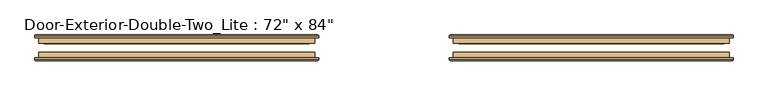
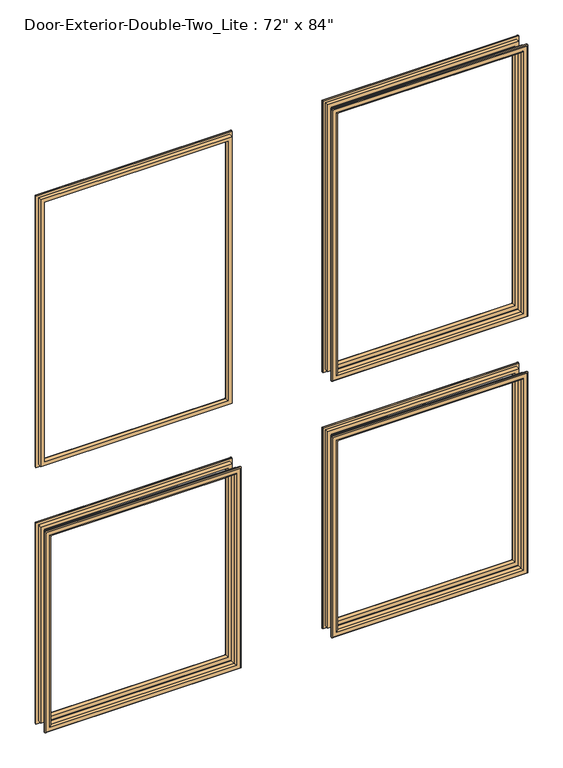
"""IFC4 building model written with IfcOpenShell, lengths in millimetres: door geometry."""

from ifc_helpers import new_model, si_unit, frame, origin, place, context, project, spatial, ellipse_curve, source, transform, mapped, element, save
from ifc_brep_helpers import plane_surface, cylinder_surface, advanced_brep


def door_a30fd648(model_context):
    return source(origin(), model_context, "Body", "AdvancedBrep", [
        advanced_brep(
        [(-762.0, 71.4375, 914.4), (-762.0, 84.1375, 914.4), (-762.0, 84.1375, 254.0), (-762.0, 71.4375, 254.0), (-750.0, 85.1375, 902.4), (-750.0, 71.4375, 902.4), (-750.0, 71.4375, 266.0), (-750.0, 85.1375, 266.0), (-755.0, 90.1375, 907.4), (-755.0, 90.1375, 261.0), (-770.0, 88.1375, 922.4), (-768.0, 90.1375, 920.4), (-768.0, 90.1375, 248.0), (-770.0, 88.1375, 246.0), (-770.0, 84.1375, 922.4), (-770.0, 84.1375, 246.0), (-152.4, 84.1375, 254.0), (-152.4, 71.4375, 254.0), (-164.4, 71.4375, 266.0), (-164.4, 85.1375, 266.0), (-159.4, 90.1375, 261.0), (-146.4, 90.1375, 248.0), (-144.4, 88.1375, 246.0), (-144.4, 84.1375, 246.0), (-152.4, 84.1375, 914.4), (-152.4, 71.4375, 914.4), (-164.4, 71.4375, 902.4), (-164.4, 85.1375, 902.4), (-159.4, 90.1375, 907.4), (-146.4, 90.1375, 920.4), (-144.4, 88.1375, 922.4), (-144.4, 84.1375, 922.4)],
        [
            (0, 1),
            (1, 2),
            (2, 3),
            (3, 0),
            (4, 5),
            (5, 6),
            (6, 7),
            (7, 4),
            (8, 4, ellipse_curve(frame((-755.0, 85.1375, 907.4), z_axis=(-0.7071067811865475, 0.0, -0.7071067811865475), x_axis=(-0.7071067811865474, 0.0, 0.7071067811865476)), 7.0710678, 5.0)),
            (7, 9, ellipse_curve(frame((-755.0, 85.1375, 261.0), z_axis=(-0.7071067811865475, 0.0, 0.7071067811865475), x_axis=(0.7071067811865474, 0.0, 0.7071067811865476)), 7.0710678, 5.0)),
            (9, 8),
            (10, 11, ellipse_curve(frame((-768.0, 88.1375, 920.4), z_axis=(-0.7071067811865475, 0.0, -0.7071067811865475), x_axis=(-0.7071067811865474, 0.0, 0.7071067811865476)), 2.8284271, 2.0)),
            (11, 12),
            (12, 13, ellipse_curve(frame((-768.0, 88.1375, 248.0), z_axis=(-0.7071067811865475, 0.0, 0.7071067811865475), x_axis=(0.7071067811865474, 0.0, 0.7071067811865476)), 2.8284271, 2.0)),
            (13, 10),
            (14, 10),
            (13, 15),
            (15, 14),
            (2, 16),
            (16, 17),
            (17, 3),
            (6, 18),
            (18, 19),
            (19, 7),
            (19, 20, ellipse_curve(frame((-159.4, 85.1375, 261.0), z_axis=(-0.7071067811865475, 0.0, -0.7071067811865475), x_axis=(-0.7071067811865476, 0.0, 0.7071067811865474)), 7.0710678, 5.0)),
            (20, 9),
            (12, 21),
            (21, 22, ellipse_curve(frame((-146.4, 88.1375, 248.0), z_axis=(-0.7071067811865475, 0.0, -0.7071067811865475), x_axis=(-0.7071067811865476, 0.0, 0.7071067811865474)), 2.8284271, 2.0)),
            (22, 13),
            (22, 23),
            (23, 15),
            (16, 24),
            (24, 25),
            (25, 17),
            (18, 26),
            (26, 27),
            (27, 19),
            (27, 28, ellipse_curve(frame((-159.4, 85.1375, 907.4), z_axis=(0.7071067811865475, 0.0, -0.7071067811865475), x_axis=(-0.7071067811865474, 0.0, -0.7071067811865476)), 7.0710678, 5.0)),
            (28, 20),
            (21, 29),
            (29, 30, ellipse_curve(frame((-146.4, 88.1375, 920.4), z_axis=(0.7071067811865475, 0.0, -0.7071067811865475), x_axis=(-0.7071067811865474, 0.0, -0.7071067811865476)), 2.8284271, 2.0)),
            (30, 22),
            (30, 31),
            (31, 23),
            (31, 14),
            (1, 24),
            (0, 25),
            (5, 26),
            (4, 27),
            (8, 28),
            (11, 29),
            (10, 30),
        ],
        [
            plane_surface(frame((-762.0, 84.1375, 914.4), z_axis=(-1.0, 0.0, 0.0), x_axis=(0.0, 0.0, -1.0))),
            plane_surface(frame((-750.0, 71.4375, 902.4), z_axis=(1.0, 0.0, 0.0), x_axis=(0.0, 0.0, -1.0))),
            cylinder_surface(frame((-755.0, 85.1375, 914.4), z_axis=(0.0, 0.0, 1.0), x_axis=(-1.0, 0.0, 0.0)), 5.0),
            cylinder_surface(frame((-768.0, 88.1375, 914.4), z_axis=(0.0, 0.0, 1.0), x_axis=(-1.0, 0.0, 0.0)), 2.0),
            plane_surface(frame((-770.0, 88.1375, 922.4), z_axis=(-1.0, 0.0, 0.0), x_axis=(0.0, 0.0, -1.0))),
            plane_surface(frame((-762.0, 84.1375, 254.0), z_axis=(0.0, 0.0, -1.0), x_axis=(1.0, 0.0, 0.0))),
            plane_surface(frame((-750.0, 71.4375, 266.0), z_axis=(0.0, 0.0, 1.0), x_axis=(1.0, 0.0, 0.0))),
            cylinder_surface(frame((-762.0, 85.1375, 261.0), z_axis=(-1.0, 0.0, 0.0), x_axis=(0.0, 0.0, -1.0)), 5.0),
            cylinder_surface(frame((-762.0, 88.1375, 248.0), z_axis=(-1.0, 0.0, 0.0), x_axis=(0.0, 0.0, -1.0)), 2.0),
            plane_surface(frame((-770.0, 88.1375, 246.0), z_axis=(0.0, 0.0, -1.0), x_axis=(1.0, 0.0, 0.0))),
            plane_surface(frame((-152.4, 84.1375, 254.0), z_axis=(1.0, 0.0, 0.0), x_axis=(0.0, 0.0, 1.0))),
            plane_surface(frame((-164.4, 71.4375, 266.0), z_axis=(-1.0, 0.0, 0.0), x_axis=(0.0, 0.0, 1.0))),
            cylinder_surface(frame((-159.4, 85.1375, 254.0), z_axis=(0.0, 0.0, -1.0), x_axis=(1.0, 0.0, 0.0)), 5.0),
            cylinder_surface(frame((-146.4, 88.1375, 254.0), z_axis=(0.0, 0.0, -1.0), x_axis=(1.0, 0.0, 0.0)), 2.0),
            plane_surface(frame((-144.4, 88.1375, 246.0), z_axis=(1.0, 0.0, 0.0), x_axis=(0.0, 0.0, 1.0))),
            plane_surface(frame((-144.4, 84.1375, 922.4), z_axis=(0.0, -1.0, 0.0), x_axis=(-1.0, 0.0, 0.0))),
            plane_surface(frame((-152.4, 84.1375, 914.4), z_axis=(0.0, 0.0, 1.0), x_axis=(-1.0, 0.0, 0.0))),
            plane_surface(frame((-152.4, 71.4375, 914.4), z_axis=(0.0, -1.0, 0.0), x_axis=(-1.0, 0.0, 0.0))),
            plane_surface(frame((-164.4, 71.4375, 902.4), z_axis=(0.0, 0.0, -1.0), x_axis=(-1.0, 0.0, 0.0))),
            cylinder_surface(frame((-152.4, 85.1375, 907.4), z_axis=(1.0, 0.0, 0.0), x_axis=(0.0, 0.0, 1.0)), 5.0),
            plane_surface(frame((-159.4, 90.1375, 907.4), z_axis=(0.0, 1.0, 0.0), x_axis=(-1.0, 0.0, 0.0))),
            cylinder_surface(frame((-152.4, 88.1375, 920.4), z_axis=(1.0, 0.0, 0.0), x_axis=(0.0, 0.0, 1.0)), 2.0),
            plane_surface(frame((-144.4, 88.1375, 922.4), z_axis=(0.0, 0.0, 1.0), x_axis=(-1.0, 0.0, 0.0))),
        ],
        [
            (0, [[1, 2, 3, 4]]),
            (1, [[5, 6, 7, 8]]),
            (2, [[9, -8, 10, 11]]),
            (3, [[12, 13, 14, 15]]),
            (4, [[16, -15, 17, 18]]),
            (5, [[-3, 19, 20, 21]]),
            (6, [[-7, 22, 23, 24]]),
            (7, [[-10, -24, 25, 26]]),
            (8, [[-14, 27, 28, 29]]),
            (9, [[-17, -29, 30, 31]]),
            (10, [[-20, 32, 33, 34]]),
            (11, [[-23, 35, 36, 37]]),
            (12, [[-25, -37, 38, 39]]),
            (13, [[-28, 40, 41, 42]]),
            (14, [[-30, -42, 43, 44]]),
            (15, [[-31, -44, 45, -18], [46, -32, -19, -2]]),
            (16, [[-33, -46, -1, 47]]),
            (17, [[-21, -34, -47, -4], [48, -35, -22, -6]]),
            (18, [[-36, -48, -5, 49]]),
            (19, [[-38, -49, -9, 50]]),
            (20, [[51, -40, -27, -13], [-26, -39, -50, -11]]),
            (21, [[-41, -51, -12, 52]]),
            (22, [[-43, -52, -16, -45]]),
        ],
    ),
        advanced_brep(
        [(152.4, 71.4375, 914.4), (152.4, 84.1375, 914.4), (152.4, 84.1375, 254.0), (152.4, 71.4375, 254.0), (164.4, 85.1375, 902.4), (164.4, 71.4375, 902.4), (164.4, 71.4375, 266.0), (164.4, 85.1375, 266.0), (159.4, 90.1375, 907.4), (159.4, 90.1375, 261.0), (144.4, 88.1375, 922.4), (146.4, 90.1375, 920.4), (146.4, 90.1375, 248.0), (144.4, 88.1375, 246.0), (144.4, 84.1375, 922.4), (144.4, 84.1375, 246.0), (762.0, 84.1375, 254.0), (762.0, 71.4375, 254.0), (750.0, 71.4375, 266.0), (750.0, 85.1375, 266.0), (755.0, 90.1375, 261.0), (768.0, 90.1375, 248.0), (770.0, 88.1375, 246.0), (770.0, 84.1375, 246.0), (762.0, 84.1375, 914.4), (762.0, 71.4375, 914.4), (750.0, 71.4375, 902.4), (750.0, 85.1375, 902.4), (755.0, 90.1375, 907.4), (768.0, 90.1375, 920.4), (770.0, 88.1375, 922.4), (770.0, 84.1375, 922.4)],
        [
            (0, 1),
            (1, 2),
            (2, 3),
            (3, 0),
            (4, 5),
            (5, 6),
            (6, 7),
            (7, 4),
            (8, 4, ellipse_curve(frame((159.4, 85.1375, 907.4), z_axis=(-0.7071067811865475, 0.0, -0.7071067811865475), x_axis=(-0.7071067811865474, 0.0, 0.7071067811865476)), 7.0710678, 5.0)),
            (7, 9, ellipse_curve(frame((159.4, 85.1375, 261.0), z_axis=(-0.7071067811865475, 0.0, 0.7071067811865475), x_axis=(0.7071067811865474, 0.0, 0.7071067811865476)), 7.0710678, 5.0)),
            (9, 8),
            (10, 11, ellipse_curve(frame((146.4, 88.1375, 920.4), z_axis=(-0.7071067811865475, 0.0, -0.7071067811865475), x_axis=(-0.7071067811865474, 0.0, 0.7071067811865476)), 2.8284271, 2.0)),
            (11, 12),
            (12, 13, ellipse_curve(frame((146.4, 88.1375, 248.0), z_axis=(-0.7071067811865475, 0.0, 0.7071067811865475), x_axis=(0.7071067811865474, 0.0, 0.7071067811865476)), 2.8284271, 2.0)),
            (13, 10),
            (14, 10),
            (13, 15),
            (15, 14),
            (2, 16),
            (16, 17),
            (17, 3),
            (6, 18),
            (18, 19),
            (19, 7),
            (19, 20, ellipse_curve(frame((755.0, 85.1375, 261.0), z_axis=(-0.7071067811865475, 0.0, -0.7071067811865475), x_axis=(-0.7071067811865476, 0.0, 0.7071067811865474)), 7.0710678, 5.0)),
            (20, 9),
            (12, 21),
            (21, 22, ellipse_curve(frame((768.0, 88.1375, 248.0), z_axis=(-0.7071067811865475, 0.0, -0.7071067811865475), x_axis=(-0.7071067811865476, 0.0, 0.7071067811865474)), 2.8284271, 2.0)),
            (22, 13),
            (22, 23),
            (23, 15),
            (16, 24),
            (24, 25),
            (25, 17),
            (18, 26),
            (26, 27),
            (27, 19),
            (27, 28, ellipse_curve(frame((755.0, 85.1375, 907.4), z_axis=(0.7071067811865475, 0.0, -0.7071067811865475), x_axis=(-0.7071067811865474, 0.0, -0.7071067811865476)), 7.0710678, 5.0)),
            (28, 20),
            (21, 29),
            (29, 30, ellipse_curve(frame((768.0, 88.1375, 920.4), z_axis=(0.7071067811865475, 0.0, -0.7071067811865475), x_axis=(-0.7071067811865474, 0.0, -0.7071067811865476)), 2.8284271, 2.0)),
            (30, 22),
            (30, 31),
            (31, 23),
            (31, 14),
            (1, 24),
            (0, 25),
            (5, 26),
            (4, 27),
            (8, 28),
            (11, 29),
            (10, 30),
        ],
        [
            plane_surface(frame((152.4, 84.1375, 914.4), z_axis=(-1.0, 0.0, 0.0), x_axis=(0.0, 0.0, -1.0))),
            plane_surface(frame((164.4, 71.4375, 902.4), z_axis=(1.0, 0.0, 0.0), x_axis=(0.0, 0.0, -1.0))),
            cylinder_surface(frame((159.4, 85.1375, 914.4), z_axis=(0.0, 0.0, 1.0), x_axis=(-1.0, 0.0, 0.0)), 5.0),
            cylinder_surface(frame((146.4, 88.1375, 914.4), z_axis=(0.0, 0.0, 1.0), x_axis=(-1.0, 0.0, 0.0)), 2.0),
            plane_surface(frame((144.4, 88.1375, 922.4), z_axis=(-1.0, 0.0, 0.0), x_axis=(0.0, 0.0, -1.0))),
            plane_surface(frame((152.4, 84.1375, 254.0), z_axis=(0.0, 0.0, -1.0), x_axis=(1.0, 0.0, 0.0))),
            plane_surface(frame((164.4, 71.4375, 266.0), z_axis=(0.0, 0.0, 1.0), x_axis=(1.0, 0.0, 0.0))),
            cylinder_surface(frame((152.4, 85.1375, 261.0), z_axis=(-1.0, 0.0, 0.0), x_axis=(0.0, 0.0, -1.0)), 5.0),
            cylinder_surface(frame((152.4, 88.1375, 248.0), z_axis=(-1.0, 0.0, 0.0), x_axis=(0.0, 0.0, -1.0)), 2.0),
            plane_surface(frame((144.4, 88.1375, 246.0), z_axis=(0.0, 0.0, -1.0), x_axis=(1.0, 0.0, 0.0))),
            plane_surface(frame((762.0, 84.1375, 254.0), z_axis=(1.0, 0.0, 0.0), x_axis=(0.0, 0.0, 1.0))),
            plane_surface(frame((750.0, 71.4375, 266.0), z_axis=(-1.0, 0.0, 0.0), x_axis=(0.0, 0.0, 1.0))),
            cylinder_surface(frame((755.0, 85.1375, 254.0), z_axis=(0.0, 0.0, -1.0), x_axis=(1.0, 0.0, 0.0)), 5.0),
            cylinder_surface(frame((768.0, 88.1375, 254.0), z_axis=(0.0, 0.0, -1.0), x_axis=(1.0, 0.0, 0.0)), 2.0),
            plane_surface(frame((770.0, 88.1375, 246.0), z_axis=(1.0, 0.0, 0.0), x_axis=(0.0, 0.0, 1.0))),
            plane_surface(frame((770.0, 84.1375, 922.4), z_axis=(0.0, -1.0, 0.0), x_axis=(-1.0, 0.0, 0.0))),
            plane_surface(frame((762.0, 84.1375, 914.4), z_axis=(0.0, 0.0, 1.0), x_axis=(-1.0, 0.0, 0.0))),
            plane_surface(frame((762.0, 71.4375, 914.4), z_axis=(0.0, -1.0, 0.0), x_axis=(-1.0, 0.0, 0.0))),
            plane_surface(frame((750.0, 71.4375, 902.4), z_axis=(0.0, 0.0, -1.0), x_axis=(-1.0, 0.0, 0.0))),
            cylinder_surface(frame((762.0, 85.1375, 907.4), z_axis=(1.0, 0.0, 0.0), x_axis=(0.0, 0.0, 1.0)), 5.0),
            plane_surface(frame((755.0, 90.1375, 907.4), z_axis=(0.0, 1.0, 0.0), x_axis=(-1.0, 0.0, 0.0))),
            cylinder_surface(frame((762.0, 88.1375, 920.4), z_axis=(1.0, 0.0, 0.0), x_axis=(0.0, 0.0, 1.0)), 2.0),
            plane_surface(frame((770.0, 88.1375, 922.4), z_axis=(0.0, 0.0, 1.0), x_axis=(-1.0, 0.0, 0.0))),
        ],
        [
            (0, [[1, 2, 3, 4]]),
            (1, [[5, 6, 7, 8]]),
            (2, [[9, -8, 10, 11]]),
            (3, [[12, 13, 14, 15]]),
            (4, [[16, -15, 17, 18]]),
            (5, [[-3, 19, 20, 21]]),
            (6, [[-7, 22, 23, 24]]),
            (7, [[-10, -24, 25, 26]]),
            (8, [[-14, 27, 28, 29]]),
            (9, [[-17, -29, 30, 31]]),
            (10, [[-20, 32, 33, 34]]),
            (11, [[-23, 35, 36, 37]]),
            (12, [[-25, -37, 38, 39]]),
            (13, [[-28, 40, 41, 42]]),
            (14, [[-30, -42, 43, 44]]),
            (15, [[-31, -44, 45, -18], [46, -32, -19, -2]]),
            (16, [[-33, -46, -1, 47]]),
            (17, [[-21, -34, -47, -4], [48, -35, -22, -6]]),
            (18, [[-36, -48, -5, 49]]),
            (19, [[-38, -49, -9, 50]]),
            (20, [[51, -40, -27, -13], [-26, -39, -50, -11]]),
            (21, [[-41, -51, -12, 52]]),
            (22, [[-43, -52, -16, -45]]),
        ],
    ),
        advanced_brep(
        [(152.4, 71.4375, 2016.125), (152.4, 84.1375, 2016.125), (152.4, 84.1375, 1117.6), (152.4, 71.4375, 1117.6), (164.4, 85.1375, 2004.125), (164.4, 71.4375, 2004.125), (164.4, 71.4375, 1129.6), (164.4, 85.1375, 1129.6), (159.4, 90.1375, 2009.125), (159.4, 90.1375, 1124.6), (144.4, 88.1375, 2024.125), (146.4, 90.1375, 2022.125), (146.4, 90.1375, 1111.6), (144.4, 88.1375, 1109.6), (144.4, 84.1375, 2024.125), (144.4, 84.1375, 1109.6), (762.0, 84.1375, 1117.6), (762.0, 71.4375, 1117.6), (750.0, 71.4375, 1129.6), (750.0, 85.1375, 1129.6), (755.0, 90.1375, 1124.6), (768.0, 90.1375, 1111.6), (770.0, 88.1375, 1109.6), (770.0, 84.1375, 1109.6), (762.0, 84.1375, 2016.125), (762.0, 71.4375, 2016.125), (750.0, 71.4375, 2004.125), (750.0, 85.1375, 2004.125), (755.0, 90.1375, 2009.125), (768.0, 90.1375, 2022.125), (770.0, 88.1375, 2024.125), (770.0, 84.1375, 2024.125)],
        [
            (0, 1),
            (1, 2),
            (2, 3),
            (3, 0),
            (4, 5),
            (5, 6),
            (6, 7),
            (7, 4),
            (8, 4, ellipse_curve(frame((159.4, 85.1375, 2009.125), z_axis=(-0.7071067811865475, 0.0, -0.7071067811865475), x_axis=(-0.7071067811865474, 0.0, 0.7071067811865476)), 7.0710678, 5.0)),
            (7, 9, ellipse_curve(frame((159.4, 85.1375, 1124.6), z_axis=(-0.7071067811865475, 0.0, 0.7071067811865475), x_axis=(0.7071067811865474, 0.0, 0.7071067811865476)), 7.0710678, 5.0)),
            (9, 8),
            (10, 11, ellipse_curve(frame((146.4, 88.1375, 2022.125), z_axis=(-0.7071067811865475, 0.0, -0.7071067811865475), x_axis=(-0.7071067811865474, 0.0, 0.7071067811865476)), 2.8284271, 2.0)),
            (11, 12),
            (12, 13, ellipse_curve(frame((146.4, 88.1375, 1111.6), z_axis=(-0.7071067811865475, 0.0, 0.7071067811865475), x_axis=(0.7071067811865474, 0.0, 0.7071067811865476)), 2.8284271, 2.0)),
            (13, 10),
            (14, 10),
            (13, 15),
            (15, 14),
            (2, 16),
            (16, 17),
            (17, 3),
            (6, 18),
            (18, 19),
            (19, 7),
            (19, 20, ellipse_curve(frame((755.0, 85.1375, 1124.6), z_axis=(-0.7071067811865475, 0.0, -0.7071067811865475), x_axis=(-0.7071067811865476, 0.0, 0.7071067811865474)), 7.0710678, 5.0)),
            (20, 9),
            (12, 21),
            (21, 22, ellipse_curve(frame((768.0, 88.1375, 1111.6), z_axis=(-0.7071067811865475, 0.0, -0.7071067811865475), x_axis=(-0.7071067811865476, 0.0, 0.7071067811865474)), 2.8284271, 2.0)),
            (22, 13),
            (22, 23),
            (23, 15),
            (16, 24),
            (24, 25),
            (25, 17),
            (18, 26),
            (26, 27),
            (27, 19),
            (27, 28, ellipse_curve(frame((755.0, 85.1375, 2009.125), z_axis=(0.7071067811865475, 0.0, -0.7071067811865475), x_axis=(-0.7071067811865474, 0.0, -0.7071067811865476)), 7.0710678, 5.0)),
            (28, 20),
            (21, 29),
            (29, 30, ellipse_curve(frame((768.0, 88.1375, 2022.125), z_axis=(0.7071067811865475, 0.0, -0.7071067811865475), x_axis=(-0.7071067811865474, 0.0, -0.7071067811865476)), 2.8284271, 2.0)),
            (30, 22),
            (30, 31),
            (31, 23),
            (31, 14),
            (1, 24),
            (0, 25),
            (5, 26),
            (4, 27),
            (8, 28),
            (11, 29),
            (10, 30),
        ],
        [
            plane_surface(frame((152.4, 84.1375, 2016.125), z_axis=(-1.0, 0.0, 0.0), x_axis=(0.0, 0.0, -1.0))),
            plane_surface(frame((164.4, 71.4375, 2004.125), z_axis=(1.0, 0.0, 0.0), x_axis=(0.0, 0.0, -1.0))),
            cylinder_surface(frame((159.4, 85.1375, 2016.125), z_axis=(0.0, 0.0, 1.0), x_axis=(-1.0, 0.0, 0.0)), 5.0),
            cylinder_surface(frame((146.4, 88.1375, 2016.125), z_axis=(0.0, 0.0, 1.0), x_axis=(-1.0, 0.0, 0.0)), 2.0),
            plane_surface(frame((144.4, 88.1375, 2024.125), z_axis=(-1.0, 0.0, 0.0), x_axis=(0.0, 0.0, -1.0))),
            plane_surface(frame((152.4, 84.1375, 1117.6), z_axis=(0.0, 0.0, -1.0), x_axis=(1.0, 0.0, 0.0))),
            plane_surface(frame((164.4, 71.4375, 1129.6), z_axis=(0.0, 0.0, 1.0), x_axis=(1.0, 0.0, 0.0))),
            cylinder_surface(frame((152.4, 85.1375, 1124.6), z_axis=(-1.0, 0.0, 0.0), x_axis=(0.0, 0.0, -1.0)), 5.0),
            cylinder_surface(frame((152.4, 88.1375, 1111.6), z_axis=(-1.0, 0.0, 0.0), x_axis=(0.0, 0.0, -1.0)), 2.0),
            plane_surface(frame((144.4, 88.1375, 1109.6), z_axis=(0.0, 0.0, -1.0), x_axis=(1.0, 0.0, 0.0))),
            plane_surface(frame((762.0, 84.1375, 1117.6), z_axis=(1.0, 0.0, 0.0), x_axis=(0.0, 0.0, 1.0))),
            plane_surface(frame((750.0, 71.4375, 1129.6), z_axis=(-1.0, 0.0, 0.0), x_axis=(0.0, 0.0, 1.0))),
            cylinder_surface(frame((755.0, 85.1375, 1117.6), z_axis=(0.0, 0.0, -1.0), x_axis=(1.0, 0.0, 0.0)), 5.0),
            cylinder_surface(frame((768.0, 88.1375, 1117.6), z_axis=(0.0, 0.0, -1.0), x_axis=(1.0, 0.0, 0.0)), 2.0),
            plane_surface(frame((770.0, 88.1375, 1109.6), z_axis=(1.0, 0.0, 0.0), x_axis=(0.0, 0.0, 1.0))),
            plane_surface(frame((770.0, 84.1375, 2024.125), z_axis=(0.0, -1.0, 0.0), x_axis=(-1.0, 0.0, 0.0))),
            plane_surface(frame((762.0, 84.1375, 2016.125), z_axis=(0.0, 0.0, 1.0), x_axis=(-1.0, 0.0, 0.0))),
            plane_surface(frame((762.0, 71.4375, 2016.125), z_axis=(0.0, -1.0, 0.0), x_axis=(-1.0, 0.0, 0.0))),
            plane_surface(frame((750.0, 71.4375, 2004.125), z_axis=(0.0, 0.0, -1.0), x_axis=(-1.0, 0.0, 0.0))),
            cylinder_surface(frame((762.0, 85.1375, 2009.125), z_axis=(1.0, 0.0, 0.0), x_axis=(0.0, 0.0, 1.0)), 5.0),
            plane_surface(frame((755.0, 90.1375, 2009.125), z_axis=(0.0, 1.0, 0.0), x_axis=(-1.0, 0.0, 0.0))),
            cylinder_surface(frame((762.0, 88.1375, 2022.125), z_axis=(1.0, 0.0, 0.0), x_axis=(0.0, 0.0, 1.0)), 2.0),
            plane_surface(frame((770.0, 88.1375, 2024.125), z_axis=(0.0, 0.0, 1.0), x_axis=(-1.0, 0.0, 0.0))),
        ],
        [
            (0, [[1, 2, 3, 4]]),
            (1, [[5, 6, 7, 8]]),
            (2, [[9, -8, 10, 11]]),
            (3, [[12, 13, 14, 15]]),
            (4, [[16, -15, 17, 18]]),
            (5, [[-3, 19, 20, 21]]),
            (6, [[-7, 22, 23, 24]]),
            (7, [[-10, -24, 25, 26]]),
            (8, [[-14, 27, 28, 29]]),
            (9, [[-17, -29, 30, 31]]),
            (10, [[-20, 32, 33, 34]]),
            (11, [[-23, 35, 36, 37]]),
            (12, [[-25, -37, 38, 39]]),
            (13, [[-28, 40, 41, 42]]),
            (14, [[-30, -42, 43, 44]]),
            (15, [[-31, -44, 45, -18], [46, -32, -19, -2]]),
            (16, [[-33, -46, -1, 47]]),
            (17, [[-21, -34, -47, -4], [48, -35, -22, -6]]),
            (18, [[-36, -48, -5, 49]]),
            (19, [[-38, -49, -9, 50]]),
            (20, [[51, -40, -27, -13], [-26, -39, -50, -11]]),
            (21, [[-41, -51, -12, 52]]),
            (22, [[-43, -52, -16, -45]]),
        ],
    ),
        advanced_brep(
        [(-762.0, 71.4375, 2016.125), (-762.0, 84.1375, 2016.125), (-762.0, 84.1375, 1117.6), (-762.0, 71.4375, 1117.6), (-750.0, 85.1375, 2004.125), (-750.0, 71.4375, 2004.125), (-750.0, 71.4375, 1129.6), (-750.0, 85.1375, 1129.6), (-755.0, 90.1375, 2009.125), (-755.0, 90.1375, 1124.6), (-770.0, 88.1375, 2024.125), (-768.0, 90.1375, 2022.125), (-768.0, 90.1375, 1111.6), (-770.0, 88.1375, 1109.6), (-770.0, 84.1375, 2024.125), (-770.0, 84.1375, 1109.6), (-152.4, 84.1375, 1117.6), (-152.4, 71.4375, 1117.6), (-164.4, 71.4375, 1129.6), (-164.4, 85.1375, 1129.6), (-159.4, 90.1375, 1124.6), (-146.4, 90.1375, 1111.6), (-144.4, 88.1375, 1109.6), (-144.4, 84.1375, 1109.6), (-152.4, 84.1375, 2016.125), (-152.4, 71.4375, 2016.125), (-164.4, 71.4375, 2004.125), (-164.4, 85.1375, 2004.125), (-159.4, 90.1375, 2009.125), (-146.4, 90.1375, 2022.125), (-144.4, 88.1375, 2024.125), (-144.4, 84.1375, 2024.125)],
        [
            (0, 1),
            (1, 2),
            (2, 3),
            (3, 0),
            (4, 5),
            (5, 6),
            (6, 7),
            (7, 4),
            (8, 4, ellipse_curve(frame((-755.0, 85.1375, 2009.125), z_axis=(-0.7071067811865475, 0.0, -0.7071067811865475), x_axis=(-0.7071067811865474, 0.0, 0.7071067811865476)), 7.0710678, 5.0)),
            (7, 9, ellipse_curve(frame((-755.0, 85.1375, 1124.6), z_axis=(-0.7071067811865475, 0.0, 0.7071067811865475), x_axis=(0.7071067811865474, 0.0, 0.7071067811865476)), 7.0710678, 5.0)),
            (9, 8),
            (10, 11, ellipse_curve(frame((-768.0, 88.1375, 2022.125), z_axis=(-0.7071067811865475, 0.0, -0.7071067811865475), x_axis=(-0.7071067811865474, 0.0, 0.7071067811865476)), 2.8284271, 2.0)),
            (11, 12),
            (12, 13, ellipse_curve(frame((-768.0, 88.1375, 1111.6), z_axis=(-0.7071067811865475, 0.0, 0.7071067811865475), x_axis=(0.7071067811865474, 0.0, 0.7071067811865476)), 2.8284271, 2.0)),
            (13, 10),
            (14, 10),
            (13, 15),
            (15, 14),
            (2, 16),
            (16, 17),
            (17, 3),
            (6, 18),
            (18, 19),
            (19, 7),
            (19, 20, ellipse_curve(frame((-159.4, 85.1375, 1124.6), z_axis=(-0.7071067811865475, 0.0, -0.7071067811865475), x_axis=(-0.7071067811865476, 0.0, 0.7071067811865474)), 7.0710678, 5.0)),
            (20, 9),
            (12, 21),
            (21, 22, ellipse_curve(frame((-146.4, 88.1375, 1111.6), z_axis=(-0.7071067811865475, 0.0, -0.7071067811865475), x_axis=(-0.7071067811865476, 0.0, 0.7071067811865474)), 2.8284271, 2.0)),
            (22, 13),
            (22, 23),
            (23, 15),
            (16, 24),
            (24, 25),
            (25, 17),
            (18, 26),
            (26, 27),
            (27, 19),
            (27, 28, ellipse_curve(frame((-159.4, 85.1375, 2009.125), z_axis=(0.7071067811865475, 0.0, -0.7071067811865475), x_axis=(-0.7071067811865474, 0.0, -0.7071067811865476)), 7.0710678, 5.0)),
            (28, 20),
            (21, 29),
            (29, 30, ellipse_curve(frame((-146.4, 88.1375, 2022.125), z_axis=(0.7071067811865475, 0.0, -0.7071067811865475), x_axis=(-0.7071067811865474, 0.0, -0.7071067811865476)), 2.8284271, 2.0)),
            (30, 22),
            (30, 31),
            (31, 23),
            (31, 14),
            (1, 24),
            (0, 25),
            (5, 26),
            (4, 27),
            (8, 28),
            (11, 29),
            (10, 30),
        ],
        [
            plane_surface(frame((-762.0, 84.1375, 2016.125), z_axis=(-1.0, 0.0, 0.0), x_axis=(0.0, 0.0, -1.0))),
            plane_surface(frame((-750.0, 71.4375, 2004.125), z_axis=(1.0, 0.0, 0.0), x_axis=(0.0, 0.0, -1.0))),
            cylinder_surface(frame((-755.0, 85.1375, 2016.125), z_axis=(0.0, 0.0, 1.0), x_axis=(-1.0, 0.0, 0.0)), 5.0),
            cylinder_surface(frame((-768.0, 88.1375, 2016.125), z_axis=(0.0, 0.0, 1.0), x_axis=(-1.0, 0.0, 0.0)), 2.0),
            plane_surface(frame((-770.0, 88.1375, 2024.125), z_axis=(-1.0, 0.0, 0.0), x_axis=(0.0, 0.0, -1.0))),
            plane_surface(frame((-762.0, 84.1375, 1117.6), z_axis=(0.0, 0.0, -1.0), x_axis=(1.0, 0.0, 0.0))),
            plane_surface(frame((-750.0, 71.4375, 1129.6), z_axis=(0.0, 0.0, 1.0), x_axis=(1.0, 0.0, 0.0))),
            cylinder_surface(frame((-762.0, 85.1375, 1124.6), z_axis=(-1.0, 0.0, 0.0), x_axis=(0.0, 0.0, -1.0)), 5.0),
            cylinder_surface(frame((-762.0, 88.1375, 1111.6), z_axis=(-1.0, 0.0, 0.0), x_axis=(0.0, 0.0, -1.0)), 2.0),
            plane_surface(frame((-770.0, 88.1375, 1109.6), z_axis=(0.0, 0.0, -1.0), x_axis=(1.0, 0.0, 0.0))),
            plane_surface(frame((-152.4, 84.1375, 1117.6), z_axis=(1.0, 0.0, 0.0), x_axis=(0.0, 0.0, 1.0))),
            plane_surface(frame((-164.4, 71.4375, 1129.6), z_axis=(-1.0, 0.0, 0.0), x_axis=(0.0, 0.0, 1.0))),
            cylinder_surface(frame((-159.4, 85.1375, 1117.6), z_axis=(0.0, 0.0, -1.0), x_axis=(1.0, 0.0, 0.0)), 5.0),
            cylinder_surface(frame((-146.4, 88.1375, 1117.6), z_axis=(0.0, 0.0, -1.0), x_axis=(1.0, 0.0, 0.0)), 2.0),
            plane_surface(frame((-144.4, 88.1375, 1109.6), z_axis=(1.0, 0.0, 0.0), x_axis=(0.0, 0.0, 1.0))),
            plane_surface(frame((-144.4, 84.1375, 2024.125), z_axis=(0.0, -1.0, 0.0), x_axis=(-1.0, 0.0, 0.0))),
            plane_surface(frame((-152.4, 84.1375, 2016.125), z_axis=(0.0, 0.0, 1.0), x_axis=(-1.0, 0.0, 0.0))),
            plane_surface(frame((-152.4, 71.4375, 2016.125), z_axis=(0.0, -1.0, 0.0), x_axis=(-1.0, 0.0, 0.0))),
            plane_surface(frame((-164.4, 71.4375, 2004.125), z_axis=(0.0, 0.0, -1.0), x_axis=(-1.0, 0.0, 0.0))),
            cylinder_surface(frame((-152.4, 85.1375, 2009.125), z_axis=(1.0, 0.0, 0.0), x_axis=(0.0, 0.0, 1.0)), 5.0),
            plane_surface(frame((-159.4, 90.1375, 2009.125), z_axis=(0.0, 1.0, 0.0), x_axis=(-1.0, 0.0, 0.0))),
            cylinder_surface(frame((-152.4, 88.1375, 2022.125), z_axis=(1.0, 0.0, 0.0), x_axis=(0.0, 0.0, 1.0)), 2.0),
            plane_surface(frame((-144.4, 88.1375, 2024.125), z_axis=(0.0, 0.0, 1.0), x_axis=(-1.0, 0.0, 0.0))),
        ],
        [
            (0, [[1, 2, 3, 4]]),
            (1, [[5, 6, 7, 8]]),
            (2, [[9, -8, 10, 11]]),
            (3, [[12, 13, 14, 15]]),
            (4, [[16, -15, 17, 18]]),
            (5, [[-3, 19, 20, 21]]),
            (6, [[-7, 22, 23, 24]]),
            (7, [[-10, -24, 25, 26]]),
            (8, [[-14, 27, 28, 29]]),
            (9, [[-17, -29, 30, 31]]),
            (10, [[-20, 32, 33, 34]]),
            (11, [[-23, 35, 36, 37]]),
            (12, [[-25, -37, 38, 39]]),
            (13, [[-28, 40, 41, 42]]),
            (14, [[-30, -42, 43, 44]]),
            (15, [[-31, -44, 45, -18], [46, -32, -19, -2]]),
            (16, [[-33, -46, -1, 47]]),
            (17, [[-21, -34, -47, -4], [48, -35, -22, -6]]),
            (18, [[-36, -48, -5, 49]]),
            (19, [[-38, -49, -9, 50]]),
            (20, [[51, -40, -27, -13], [-26, -39, -50, -11]]),
            (21, [[-41, -51, -12, 52]]),
            (22, [[-43, -52, -16, -45]]),
        ],
    ),
        advanced_brep(
        [(-762.0, 52.3875, 254.0), (-762.0, 39.6875, 254.0), (-762.0, 39.6875, 914.4), (-762.0, 52.3875, 914.4), (-750.0, 38.6875, 266.0), (-750.0, 52.3875, 266.0), (-750.0, 52.3875, 902.4), (-750.0, 38.6875, 902.4), (-755.0, 33.6875, 261.0), (-755.0, 33.6875, 907.4), (-770.0, 35.6875, 246.0), (-768.0, 33.6875, 248.0), (-768.0, 33.6875, 920.4), (-770.0, 35.6875, 922.4), (-770.0, 39.6875, 246.0), (-770.0, 39.6875, 922.4), (-152.4, 39.6875, 914.4), (-152.4, 52.3875, 914.4), (-164.4, 52.3875, 902.4), (-164.4, 38.6875, 902.4), (-159.4, 33.6875, 907.4), (-146.4, 33.6875, 920.4), (-144.4, 35.6875, 922.4), (-144.4, 39.6875, 922.4), (-152.4, 39.6875, 254.0), (-152.4, 52.3875, 254.0), (-164.4, 52.3875, 266.0), (-164.4, 38.6875, 266.0), (-159.4, 33.6875, 261.0), (-146.4, 33.6875, 248.0), (-144.4, 35.6875, 246.0), (-144.4, 39.6875, 246.0)],
        [
            (0, 1),
            (1, 2),
            (2, 3),
            (3, 0),
            (4, 5),
            (5, 6),
            (6, 7),
            (7, 4),
            (8, 4, ellipse_curve(frame((-755.0, 38.6875, 261.0), z_axis=(-0.7071067811865475, 0.0, 0.7071067811865475), x_axis=(-0.7071067811865474, 0.0, -0.7071067811865476)), 7.0710678, 5.0)),
            (7, 9, ellipse_curve(frame((-755.0, 38.6875, 907.4), z_axis=(-0.7071067811865475, 0.0, -0.7071067811865475), x_axis=(0.7071067811865474, 0.0, -0.7071067811865476)), 7.0710678, 5.0)),
            (9, 8),
            (10, 11, ellipse_curve(frame((-768.0, 35.6875, 248.0), z_axis=(-0.7071067811865475, 0.0, 0.7071067811865475), x_axis=(-0.7071067811865474, 0.0, -0.7071067811865476)), 2.8284271, 2.0)),
            (11, 12),
            (12, 13, ellipse_curve(frame((-768.0, 35.6875, 920.4), z_axis=(-0.7071067811865475, 0.0, -0.7071067811865475), x_axis=(0.7071067811865474, 0.0, -0.7071067811865476)), 2.8284271, 2.0)),
            (13, 10),
            (14, 10),
            (13, 15),
            (15, 14),
            (2, 16),
            (16, 17),
            (17, 3),
            (6, 18),
            (18, 19),
            (19, 7),
            (19, 20, ellipse_curve(frame((-159.4, 38.6875, 907.4), z_axis=(-0.7071067811865475, 0.0, 0.7071067811865475), x_axis=(-0.7071067811865476, 0.0, -0.7071067811865474)), 7.0710678, 5.0)),
            (20, 9),
            (12, 21),
            (21, 22, ellipse_curve(frame((-146.4, 35.6875, 920.4), z_axis=(-0.7071067811865475, 0.0, 0.7071067811865475), x_axis=(-0.7071067811865476, 0.0, -0.7071067811865474)), 2.8284271, 2.0)),
            (22, 13),
            (22, 23),
            (23, 15),
            (16, 24),
            (24, 25),
            (25, 17),
            (18, 26),
            (26, 27),
            (27, 19),
            (27, 28, ellipse_curve(frame((-159.4, 38.6875, 261.0), z_axis=(0.7071067811865475, 0.0, 0.7071067811865475), x_axis=(-0.7071067811865474, 0.0, 0.7071067811865476)), 7.0710678, 5.0)),
            (28, 20),
            (21, 29),
            (29, 30, ellipse_curve(frame((-146.4, 35.6875, 248.0), z_axis=(0.7071067811865475, 0.0, 0.7071067811865475), x_axis=(-0.7071067811865474, 0.0, 0.7071067811865476)), 2.8284271, 2.0)),
            (30, 22),
            (30, 31),
            (31, 23),
            (31, 14),
            (1, 24),
            (0, 25),
            (5, 26),
            (4, 27),
            (8, 28),
            (11, 29),
            (10, 30),
        ],
        [
            plane_surface(frame((-762.0, 39.6875, 254.0), z_axis=(-1.0, 0.0, 0.0), x_axis=(0.0, 0.0, 1.0))),
            plane_surface(frame((-750.0, 52.3875, 266.0), z_axis=(1.0, 0.0, 0.0), x_axis=(0.0, 0.0, 1.0))),
            cylinder_surface(frame((-755.0, 38.6875, 254.0), z_axis=(0.0, 0.0, -1.0), x_axis=(-1.0, 0.0, 0.0)), 5.0),
            cylinder_surface(frame((-768.0, 35.6875, 254.0), z_axis=(0.0, 0.0, -1.0), x_axis=(-1.0, 0.0, 0.0)), 2.0),
            plane_surface(frame((-770.0, 35.6875, 246.0), z_axis=(-1.0, 0.0, 0.0), x_axis=(0.0, 0.0, 1.0))),
            plane_surface(frame((-762.0, 39.6875, 914.4), z_axis=(0.0, 0.0, 1.0), x_axis=(1.0, 0.0, 0.0))),
            plane_surface(frame((-750.0, 52.3875, 902.4), z_axis=(0.0, 0.0, -1.0), x_axis=(1.0, 0.0, 0.0))),
            cylinder_surface(frame((-762.0, 38.6875, 907.4), z_axis=(-1.0, 0.0, 0.0), x_axis=(0.0, 0.0, 1.0)), 5.0),
            cylinder_surface(frame((-762.0, 35.6875, 920.4), z_axis=(-1.0, 0.0, 0.0), x_axis=(0.0, 0.0, 1.0)), 2.0),
            plane_surface(frame((-770.0, 35.6875, 922.4), z_axis=(0.0, 0.0, 1.0), x_axis=(1.0, 0.0, 0.0))),
            plane_surface(frame((-152.4, 39.6875, 914.4), z_axis=(1.0, 0.0, 0.0), x_axis=(0.0, 0.0, -1.0))),
            plane_surface(frame((-164.4, 52.3875, 902.4), z_axis=(-1.0, 0.0, 0.0), x_axis=(0.0, 0.0, -1.0))),
            cylinder_surface(frame((-159.4, 38.6875, 914.4), z_axis=(0.0, 0.0, 1.0), x_axis=(1.0, 0.0, 0.0)), 5.0),
            cylinder_surface(frame((-146.4, 35.6875, 914.4), z_axis=(0.0, 0.0, 1.0), x_axis=(1.0, 0.0, 0.0)), 2.0),
            plane_surface(frame((-144.4, 35.6875, 922.4), z_axis=(1.0, 0.0, 0.0), x_axis=(0.0, 0.0, -1.0))),
            plane_surface(frame((-144.4, 39.6875, 246.0), z_axis=(0.0, 1.0, 0.0), x_axis=(-1.0, 0.0, 0.0))),
            plane_surface(frame((-152.4, 39.6875, 254.0), z_axis=(0.0, 0.0, -1.0), x_axis=(-1.0, 0.0, 0.0))),
            plane_surface(frame((-152.4, 52.3875, 254.0), z_axis=(0.0, 1.0, 0.0), x_axis=(-1.0, 0.0, 0.0))),
            plane_surface(frame((-164.4, 52.3875, 266.0), z_axis=(0.0, 0.0, 1.0), x_axis=(-1.0, 0.0, 0.0))),
            cylinder_surface(frame((-152.4, 38.6875, 261.0), z_axis=(1.0, 0.0, 0.0), x_axis=(0.0, 0.0, -1.0)), 5.0),
            plane_surface(frame((-159.4, 33.6875, 261.0), z_axis=(0.0, -1.0, 0.0), x_axis=(-1.0, 0.0, 0.0))),
            cylinder_surface(frame((-152.4, 35.6875, 248.0), z_axis=(1.0, 0.0, 0.0), x_axis=(0.0, 0.0, -1.0)), 2.0),
            plane_surface(frame((-144.4, 35.6875, 246.0), z_axis=(0.0, 0.0, -1.0), x_axis=(-1.0, 0.0, 0.0))),
        ],
        [
            (0, [[1, 2, 3, 4]]),
            (1, [[5, 6, 7, 8]]),
            (2, [[9, -8, 10, 11]]),
            (3, [[12, 13, 14, 15]]),
            (4, [[16, -15, 17, 18]]),
            (5, [[-3, 19, 20, 21]]),
            (6, [[-7, 22, 23, 24]]),
            (7, [[-10, -24, 25, 26]]),
            (8, [[-14, 27, 28, 29]]),
            (9, [[-17, -29, 30, 31]]),
            (10, [[-20, 32, 33, 34]]),
            (11, [[-23, 35, 36, 37]]),
            (12, [[-25, -37, 38, 39]]),
            (13, [[-28, 40, 41, 42]]),
            (14, [[-30, -42, 43, 44]]),
            (15, [[-31, -44, 45, -18], [46, -32, -19, -2]]),
            (16, [[-33, -46, -1, 47]]),
            (17, [[-21, -34, -47, -4], [48, -35, -22, -6]]),
            (18, [[-36, -48, -5, 49]]),
            (19, [[-38, -49, -9, 50]]),
            (20, [[51, -40, -27, -13], [-26, -39, -50, -11]]),
            (21, [[-41, -51, -12, 52]]),
            (22, [[-43, -52, -16, -45]]),
        ],
    ),
        advanced_brep(
        [(152.4, 52.3875, 254.0), (152.4, 39.6875, 254.0), (152.4, 39.6875, 914.4), (152.4, 52.3875, 914.4), (164.4, 38.6875, 266.0), (164.4, 52.3875, 266.0), (164.4, 52.3875, 902.4), (164.4, 38.6875, 902.4), (159.4, 33.6875, 261.0), (159.4, 33.6875, 907.4), (144.4, 35.6875, 246.0), (146.4, 33.6875, 248.0), (146.4, 33.6875, 920.4), (144.4, 35.6875, 922.4), (144.4, 39.6875, 246.0), (144.4, 39.6875, 922.4), (762.0, 39.6875, 914.4), (762.0, 52.3875, 914.4), (750.0, 52.3875, 902.4), (750.0, 38.6875, 902.4), (755.0, 33.6875, 907.4), (768.0, 33.6875, 920.4), (770.0, 35.6875, 922.4), (770.0, 39.6875, 922.4), (762.0, 39.6875, 254.0), (762.0, 52.3875, 254.0), (750.0, 52.3875, 266.0), (750.0, 38.6875, 266.0), (755.0, 33.6875, 261.0), (768.0, 33.6875, 248.0), (770.0, 35.6875, 246.0), (770.0, 39.6875, 246.0)],
        [
            (0, 1),
            (1, 2),
            (2, 3),
            (3, 0),
            (4, 5),
            (5, 6),
            (6, 7),
            (7, 4),
            (8, 4, ellipse_curve(frame((159.4, 38.6875, 261.0), z_axis=(-0.7071067811865475, 0.0, 0.7071067811865475), x_axis=(-0.7071067811865474, 0.0, -0.7071067811865476)), 7.0710678, 5.0)),
            (7, 9, ellipse_curve(frame((159.4, 38.6875, 907.4), z_axis=(-0.7071067811865475, 0.0, -0.7071067811865475), x_axis=(0.7071067811865474, 0.0, -0.7071067811865476)), 7.0710678, 5.0)),
            (9, 8),
            (10, 11, ellipse_curve(frame((146.4, 35.6875, 248.0), z_axis=(-0.7071067811865475, 0.0, 0.7071067811865475), x_axis=(-0.7071067811865474, 0.0, -0.7071067811865476)), 2.8284271, 2.0)),
            (11, 12),
            (12, 13, ellipse_curve(frame((146.4, 35.6875, 920.4), z_axis=(-0.7071067811865475, 0.0, -0.7071067811865475), x_axis=(0.7071067811865474, 0.0, -0.7071067811865476)), 2.8284271, 2.0)),
            (13, 10),
            (14, 10),
            (13, 15),
            (15, 14),
            (2, 16),
            (16, 17),
            (17, 3),
            (6, 18),
            (18, 19),
            (19, 7),
            (19, 20, ellipse_curve(frame((755.0, 38.6875, 907.4), z_axis=(-0.7071067811865475, 0.0, 0.7071067811865475), x_axis=(-0.7071067811865476, 0.0, -0.7071067811865474)), 7.0710678, 5.0)),
            (20, 9),
            (12, 21),
            (21, 22, ellipse_curve(frame((768.0, 35.6875, 920.4), z_axis=(-0.7071067811865475, 0.0, 0.7071067811865475), x_axis=(-0.7071067811865476, 0.0, -0.7071067811865474)), 2.8284271, 2.0)),
            (22, 13),
            (22, 23),
            (23, 15),
            (16, 24),
            (24, 25),
            (25, 17),
            (18, 26),
            (26, 27),
            (27, 19),
            (27, 28, ellipse_curve(frame((755.0, 38.6875, 261.0), z_axis=(0.7071067811865475, 0.0, 0.7071067811865475), x_axis=(-0.7071067811865474, 0.0, 0.7071067811865476)), 7.0710678, 5.0)),
            (28, 20),
            (21, 29),
            (29, 30, ellipse_curve(frame((768.0, 35.6875, 248.0), z_axis=(0.7071067811865475, 0.0, 0.7071067811865475), x_axis=(-0.7071067811865474, 0.0, 0.7071067811865476)), 2.8284271, 2.0)),
            (30, 22),
            (30, 31),
            (31, 23),
            (31, 14),
            (1, 24),
            (0, 25),
            (5, 26),
            (4, 27),
            (8, 28),
            (11, 29),
            (10, 30),
        ],
        [
            plane_surface(frame((152.4, 39.6875, 254.0), z_axis=(-1.0, 0.0, 0.0), x_axis=(0.0, 0.0, 1.0))),
            plane_surface(frame((164.4, 52.3875, 266.0), z_axis=(1.0, 0.0, 0.0), x_axis=(0.0, 0.0, 1.0))),
            cylinder_surface(frame((159.4, 38.6875, 254.0), z_axis=(0.0, 0.0, -1.0), x_axis=(-1.0, 0.0, 0.0)), 5.0),
            cylinder_surface(frame((146.4, 35.6875, 254.0), z_axis=(0.0, 0.0, -1.0), x_axis=(-1.0, 0.0, 0.0)), 2.0),
            plane_surface(frame((144.4, 35.6875, 246.0), z_axis=(-1.0, 0.0, 0.0), x_axis=(0.0, 0.0, 1.0))),
            plane_surface(frame((152.4, 39.6875, 914.4), z_axis=(0.0, 0.0, 1.0), x_axis=(1.0, 0.0, 0.0))),
            plane_surface(frame((164.4, 52.3875, 902.4), z_axis=(0.0, 0.0, -1.0), x_axis=(1.0, 0.0, 0.0))),
            cylinder_surface(frame((152.4, 38.6875, 907.4), z_axis=(-1.0, 0.0, 0.0), x_axis=(0.0, 0.0, 1.0)), 5.0),
            cylinder_surface(frame((152.4, 35.6875, 920.4), z_axis=(-1.0, 0.0, 0.0), x_axis=(0.0, 0.0, 1.0)), 2.0),
            plane_surface(frame((144.4, 35.6875, 922.4), z_axis=(0.0, 0.0, 1.0), x_axis=(1.0, 0.0, 0.0))),
            plane_surface(frame((762.0, 39.6875, 914.4), z_axis=(1.0, 0.0, 0.0), x_axis=(0.0, 0.0, -1.0))),
            plane_surface(frame((750.0, 52.3875, 902.4), z_axis=(-1.0, 0.0, 0.0), x_axis=(0.0, 0.0, -1.0))),
            cylinder_surface(frame((755.0, 38.6875, 914.4), z_axis=(0.0, 0.0, 1.0), x_axis=(1.0, 0.0, 0.0)), 5.0),
            cylinder_surface(frame((768.0, 35.6875, 914.4), z_axis=(0.0, 0.0, 1.0), x_axis=(1.0, 0.0, 0.0)), 2.0),
            plane_surface(frame((770.0, 35.6875, 922.4), z_axis=(1.0, 0.0, 0.0), x_axis=(0.0, 0.0, -1.0))),
            plane_surface(frame((770.0, 39.6875, 246.0), z_axis=(0.0, 1.0, 0.0), x_axis=(-1.0, 0.0, 0.0))),
            plane_surface(frame((762.0, 39.6875, 254.0), z_axis=(0.0, 0.0, -1.0), x_axis=(-1.0, 0.0, 0.0))),
            plane_surface(frame((762.0, 52.3875, 254.0), z_axis=(0.0, 1.0, 0.0), x_axis=(-1.0, 0.0, 0.0))),
            plane_surface(frame((750.0, 52.3875, 266.0), z_axis=(0.0, 0.0, 1.0), x_axis=(-1.0, 0.0, 0.0))),
            cylinder_surface(frame((762.0, 38.6875, 261.0), z_axis=(1.0, 0.0, 0.0), x_axis=(0.0, 0.0, -1.0)), 5.0),
            plane_surface(frame((755.0, 33.6875, 261.0), z_axis=(0.0, -1.0, 0.0), x_axis=(-1.0, 0.0, 0.0))),
            cylinder_surface(frame((762.0, 35.6875, 248.0), z_axis=(1.0, 0.0, 0.0), x_axis=(0.0, 0.0, -1.0)), 2.0),
            plane_surface(frame((770.0, 35.6875, 246.0), z_axis=(0.0, 0.0, -1.0), x_axis=(-1.0, 0.0, 0.0))),
        ],
        [
            (0, [[1, 2, 3, 4]]),
            (1, [[5, 6, 7, 8]]),
            (2, [[9, -8, 10, 11]]),
            (3, [[12, 13, 14, 15]]),
            (4, [[16, -15, 17, 18]]),
            (5, [[-3, 19, 20, 21]]),
            (6, [[-7, 22, 23, 24]]),
            (7, [[-10, -24, 25, 26]]),
            (8, [[-14, 27, 28, 29]]),
            (9, [[-17, -29, 30, 31]]),
            (10, [[-20, 32, 33, 34]]),
            (11, [[-23, 35, 36, 37]]),
            (12, [[-25, -37, 38, 39]]),
            (13, [[-28, 40, 41, 42]]),
            (14, [[-30, -42, 43, 44]]),
            (15, [[-31, -44, 45, -18], [46, -32, -19, -2]]),
            (16, [[-33, -46, -1, 47]]),
            (17, [[-21, -34, -47, -4], [48, -35, -22, -6]]),
            (18, [[-36, -48, -5, 49]]),
            (19, [[-38, -49, -9, 50]]),
            (20, [[51, -40, -27, -13], [-26, -39, -50, -11]]),
            (21, [[-41, -51, -12, 52]]),
            (22, [[-43, -52, -16, -45]]),
        ],
    ),
        advanced_brep(
        [(152.4, 52.3875, 1117.6), (152.4, 39.6875, 1117.6), (152.4, 39.6875, 2016.125), (152.4, 52.3875, 2016.125), (164.4, 38.6875, 1129.6), (164.4, 52.3875, 1129.6), (164.4, 52.3875, 2004.125), (164.4, 38.6875, 2004.125), (159.4, 33.6875, 1124.6), (159.4, 33.6875, 2009.125), (144.4, 35.6875, 1109.6), (146.4, 33.6875, 1111.6), (146.4, 33.6875, 2022.125), (144.4, 35.6875, 2024.125), (144.4, 39.6875, 1109.6), (144.4, 39.6875, 2024.125), (762.0, 39.6875, 2016.125), (762.0, 52.3875, 2016.125), (750.0, 52.3875, 2004.125), (750.0, 38.6875, 2004.125), (755.0, 33.6875, 2009.125), (768.0, 33.6875, 2022.125), (770.0, 35.6875, 2024.125), (770.0, 39.6875, 2024.125), (762.0, 39.6875, 1117.6), (762.0, 52.3875, 1117.6), (750.0, 52.3875, 1129.6), (750.0, 38.6875, 1129.6), (755.0, 33.6875, 1124.6), (768.0, 33.6875, 1111.6), (770.0, 35.6875, 1109.6), (770.0, 39.6875, 1109.6)],
        [
            (0, 1),
            (1, 2),
            (2, 3),
            (3, 0),
            (4, 5),
            (5, 6),
            (6, 7),
            (7, 4),
            (8, 4, ellipse_curve(frame((159.4, 38.6875, 1124.6), z_axis=(-0.7071067811865475, 0.0, 0.7071067811865475), x_axis=(-0.7071067811865474, 0.0, -0.7071067811865476)), 7.0710678, 5.0)),
            (7, 9, ellipse_curve(frame((159.4, 38.6875, 2009.125), z_axis=(-0.7071067811865475, 0.0, -0.7071067811865475), x_axis=(0.7071067811865474, 0.0, -0.7071067811865476)), 7.0710678, 5.0)),
            (9, 8),
            (10, 11, ellipse_curve(frame((146.4, 35.6875, 1111.6), z_axis=(-0.7071067811865475, 0.0, 0.7071067811865475), x_axis=(-0.7071067811865474, 0.0, -0.7071067811865476)), 2.8284271, 2.0)),
            (11, 12),
            (12, 13, ellipse_curve(frame((146.4, 35.6875, 2022.125), z_axis=(-0.7071067811865475, 0.0, -0.7071067811865475), x_axis=(0.7071067811865474, 0.0, -0.7071067811865476)), 2.8284271, 2.0)),
            (13, 10),
            (14, 10),
            (13, 15),
            (15, 14),
            (2, 16),
            (16, 17),
            (17, 3),
            (6, 18),
            (18, 19),
            (19, 7),
            (19, 20, ellipse_curve(frame((755.0, 38.6875, 2009.125), z_axis=(-0.7071067811865475, 0.0, 0.7071067811865475), x_axis=(-0.7071067811865476, 0.0, -0.7071067811865474)), 7.0710678, 5.0)),
            (20, 9),
            (12, 21),
            (21, 22, ellipse_curve(frame((768.0, 35.6875, 2022.125), z_axis=(-0.7071067811865475, 0.0, 0.7071067811865475), x_axis=(-0.7071067811865476, 0.0, -0.7071067811865474)), 2.8284271, 2.0)),
            (22, 13),
            (22, 23),
            (23, 15),
            (16, 24),
            (24, 25),
            (25, 17),
            (18, 26),
            (26, 27),
            (27, 19),
            (27, 28, ellipse_curve(frame((755.0, 38.6875, 1124.6), z_axis=(0.7071067811865475, 0.0, 0.7071067811865475), x_axis=(-0.7071067811865474, 0.0, 0.7071067811865476)), 7.0710678, 5.0)),
            (28, 20),
            (21, 29),
            (29, 30, ellipse_curve(frame((768.0, 35.6875, 1111.6), z_axis=(0.7071067811865475, 0.0, 0.7071067811865475), x_axis=(-0.7071067811865474, 0.0, 0.7071067811865476)), 2.8284271, 2.0)),
            (30, 22),
            (30, 31),
            (31, 23),
            (31, 14),
            (1, 24),
            (0, 25),
            (5, 26),
            (4, 27),
            (8, 28),
            (11, 29),
            (10, 30),
        ],
        [
            plane_surface(frame((152.4, 39.6875, 1117.6), z_axis=(-1.0, 0.0, 0.0), x_axis=(0.0, 0.0, 1.0))),
            plane_surface(frame((164.4, 52.3875, 1129.6), z_axis=(1.0, 0.0, 0.0), x_axis=(0.0, 0.0, 1.0))),
            cylinder_surface(frame((159.4, 38.6875, 1117.6), z_axis=(0.0, 0.0, -1.0), x_axis=(-1.0, 0.0, 0.0)), 5.0),
            cylinder_surface(frame((146.4, 35.6875, 1117.6), z_axis=(0.0, 0.0, -1.0), x_axis=(-1.0, 0.0, 0.0)), 2.0),
            plane_surface(frame((144.4, 35.6875, 1109.6), z_axis=(-1.0, 0.0, 0.0), x_axis=(0.0, 0.0, 1.0))),
            plane_surface(frame((152.4, 39.6875, 2016.125), z_axis=(0.0, 0.0, 1.0), x_axis=(1.0, 0.0, 0.0))),
            plane_surface(frame((164.4, 52.3875, 2004.125), z_axis=(0.0, 0.0, -1.0), x_axis=(1.0, 0.0, 0.0))),
            cylinder_surface(frame((152.4, 38.6875, 2009.125), z_axis=(-1.0, 0.0, 0.0), x_axis=(0.0, 0.0, 1.0)), 5.0),
            cylinder_surface(frame((152.4, 35.6875, 2022.125), z_axis=(-1.0, 0.0, 0.0), x_axis=(0.0, 0.0, 1.0)), 2.0),
            plane_surface(frame((144.4, 35.6875, 2024.125), z_axis=(0.0, 0.0, 1.0), x_axis=(1.0, 0.0, 0.0))),
            plane_surface(frame((762.0, 39.6875, 2016.125), z_axis=(1.0, 0.0, 0.0), x_axis=(0.0, 0.0, -1.0))),
            plane_surface(frame((750.0, 52.3875, 2004.125), z_axis=(-1.0, 0.0, 0.0), x_axis=(0.0, 0.0, -1.0))),
            cylinder_surface(frame((755.0, 38.6875, 2016.125), z_axis=(0.0, 0.0, 1.0), x_axis=(1.0, 0.0, 0.0)), 5.0),
            cylinder_surface(frame((768.0, 35.6875, 2016.125), z_axis=(0.0, 0.0, 1.0), x_axis=(1.0, 0.0, 0.0)), 2.0),
            plane_surface(frame((770.0, 35.6875, 2024.125), z_axis=(1.0, 0.0, 0.0), x_axis=(0.0, 0.0, -1.0))),
            plane_surface(frame((770.0, 39.6875, 1109.6), z_axis=(0.0, 1.0, 0.0), x_axis=(-1.0, 0.0, 0.0))),
            plane_surface(frame((762.0, 39.6875, 1117.6), z_axis=(0.0, 0.0, -1.0), x_axis=(-1.0, 0.0, 0.0))),
            plane_surface(frame((762.0, 52.3875, 1117.6), z_axis=(0.0, 1.0, 0.0), x_axis=(-1.0, 0.0, 0.0))),
            plane_surface(frame((750.0, 52.3875, 1129.6), z_axis=(0.0, 0.0, 1.0), x_axis=(-1.0, 0.0, 0.0))),
            cylinder_surface(frame((762.0, 38.6875, 1124.6), z_axis=(1.0, 0.0, 0.0), x_axis=(0.0, 0.0, -1.0)), 5.0),
            plane_surface(frame((755.0, 33.6875, 1124.6), z_axis=(0.0, -1.0, 0.0), x_axis=(-1.0, 0.0, 0.0))),
            cylinder_surface(frame((762.0, 35.6875, 1111.6), z_axis=(1.0, 0.0, 0.0), x_axis=(0.0, 0.0, -1.0)), 2.0),
            plane_surface(frame((770.0, 35.6875, 1109.6), z_axis=(0.0, 0.0, -1.0), x_axis=(-1.0, 0.0, 0.0))),
        ],
        [
            (0, [[1, 2, 3, 4]]),
            (1, [[5, 6, 7, 8]]),
            (2, [[9, -8, 10, 11]]),
            (3, [[12, 13, 14, 15]]),
            (4, [[16, -15, 17, 18]]),
            (5, [[-3, 19, 20, 21]]),
            (6, [[-7, 22, 23, 24]]),
            (7, [[-10, -24, 25, 26]]),
            (8, [[-14, 27, 28, 29]]),
            (9, [[-17, -29, 30, 31]]),
            (10, [[-20, 32, 33, 34]]),
            (11, [[-23, 35, 36, 37]]),
            (12, [[-25, -37, 38, 39]]),
            (13, [[-28, 40, 41, 42]]),
            (14, [[-30, -42, 43, 44]]),
            (15, [[-31, -44, 45, -18], [46, -32, -19, -2]]),
            (16, [[-33, -46, -1, 47]]),
            (17, [[-21, -34, -47, -4], [48, -35, -22, -6]]),
            (18, [[-36, -48, -5, 49]]),
            (19, [[-38, -49, -9, 50]]),
            (20, [[51, -40, -27, -13], [-26, -39, -50, -11]]),
            (21, [[-41, -51, -12, 52]]),
            (22, [[-43, -52, -16, -45]]),
        ],
    ),
    ])


if __name__ == "__main__":
    model = new_model("IFC4")
    model_context = context("Model", 3, world=origin())
    ifc_project = project(units=[si_unit("LENGTHUNIT", "METRE", prefix="MILLI")], contexts=[model_context])
    site = spatial("IfcSite", under=ifc_project)
    building = spatial("IfcBuilding", under=site)
    placement = place(None, origin())
    door_shape = door_a30fd648(model_context)
    element("IfcDoor", 1, ObjectType="Door-Exterior-Double-Two_Lite : 72\" x 84\"", at=placement, inside=building, context=model_context, shape_type="MappedRepresentation", body=[
        mapped(door_shape, transform((0.0, 0.0, 0.0), x_axis=(1.0, 0.0, 0.0), y_axis=(0.0, 1.0, 0.0), z_axis=(0.0, 0.0, 1.0))),
    ])
    save(model, "model.ifc")

# Revit data of these elements
# Type "Door-Exterior-Double-Two_Lite : 72\" x 84\""
#   Type Mark = "20"
#   Assembly Code = "B2030100"
#   Analytic Construction = "Metal frame, double glass door"
#   Top Rail = 0' - 4 5/8"
#   Threshold Length [instance default] = 6' - 4"
#   Threshold Offset [instance default] = 0' - 0 1/2"
#   Thickness = 0' - 1 3/4"
#   Thermal Resistance (R) = 1.3794 (h·ft²·°F)/BTU
#   Swing Angle [instance default] = 90.00°
#   Strike Height = 3' - 4"
#   Stiles = 0' - 6"
#   SinglePanelWidth = 3' - 0"
#   Rough Width [instance default] = 6' - 4"
#   Rough Height [instance default] = 7' - 4"
#   MFOpeningHeight [instance default] = 0' - 4"
#   MFOpeningWidth [instance default] = 0' - 4"
#   Lock Rail = 0' - 8"
#   Inset Calculate [instance default] = 0' - 4"
#   Masonry Inset [instance default] = 0' - 1"
#   Height = 7' - 0"
#   Width = 6' - 0"
#   Heat Transfer Coefficient (U) = 0.7250 BTU/(h·ft²·°F)
#   Glass Thickness = 0' - 0 3/4"
#   Masonry Frame Depth = 0' - 5 3/4"
#   Bottom Rail = 0' - 10"
#   Threshold [instance default] = yes
#   Masonry Frame [instance default] = yes
#   Function = 1
#   Dry Wall Frame [instance default] = no
#   Threshold Material = none
#   Panic Bar Material = Metal - Stainless Steel
#   Panel Material = Metal - Painted - Grey
#   Glass Stop Material = Metal - Painted - Grey
#   Frame Material = Metal - Painted - Grey
#   Exterior Pull Material = Metal - Stainless Steel
#   Visual Light Transmittance = 0
#   Solar Heat Gain Coefficient = 0
#   Wall Closure = (empty or 0)
# Element 1 (IfcDoor, "Door-Exterior-Double-Two_Lite : 72\" x 84\"")
#   Threshold Length = 6' - 0"
#   Rough Width = 6' - 2 1/2"
#   Rough Height = 7' - 1 1/4"
#   MFOpeningHeight = 0' - 1 1/4"
#   MFOpeningWidth = 0' - 2 1/2"
#   Inset Calculate = 0' - 3"
#   Masonry Frame = no
#   Dry Wall Frame = yes
#   Materials on its faces: "Metal - Painted - Grey", "Metal - Stainless Steel", "Glass"
# Materials
#   "Metal - Stainless Steel": class "Metal", colour RGB 247 247 247, transparency 0
#   "Metal - Painted - Grey": class "Paint", colour RGB 104 104 104, transparency 0, Cost = 0
#   "Glass": class "Glass", colour RGB 0 128 192, transparency 0.75, Description = "Soda Lime Glass", Cost = 0
